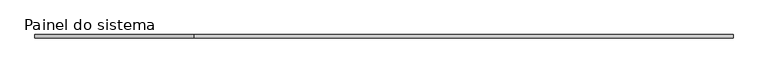
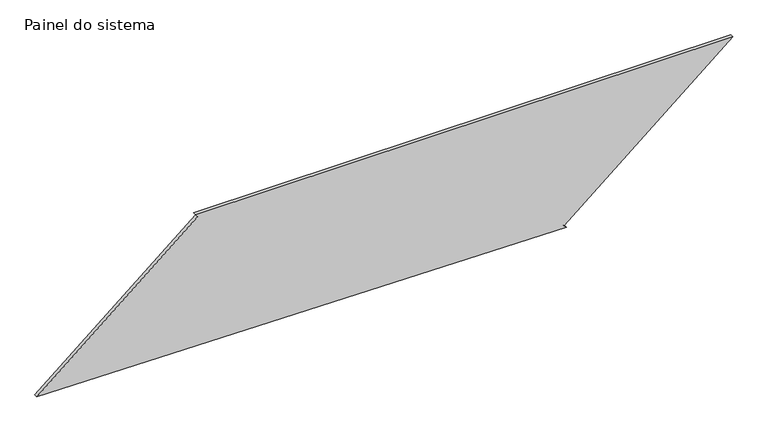
"""IFC4 building model written with IfcOpenShell, lengths in millimetres: plate geometry, Painel do sistema : Envidraçado."""

from ifc_helpers import new_model, si_unit, frame, origin, place, context, project, spatial, polyline, outline, extrude, source, transform, mapped, element, save


def painel_do_sistema_b5e3f343(model_context):
    return source(origin(), model_context, "Body", "SweptSolid", [
        extrude(outline(polyline([(0.0, 1345.1193014), (19.2037959, 1329.1126083), (1059.6226392, 2577.3398982), (1059.6226392, -1401.6658317), (1040.4188433, -1385.6591386), (47.1325024, -2577.3398982), (0.0, 1345.1193014)])), frame((0.0, 24.5, 0.0), z_axis=(0.0, 1.0, 0.0), x_axis=(0.0, 0.0, 1.0)), (0.0, 0.0, 1.0), 25.0),
    ])


if __name__ == "__main__":
    model = new_model("IFC4")
    model_context = context("Model", 3, world=origin())
    ifc_project = project(units=[si_unit("LENGTHUNIT", "METRE", prefix="MILLI")], contexts=[model_context])
    site = spatial("IfcSite", under=ifc_project)
    building = spatial("IfcBuilding", under=site)
    placement = place(None, origin())
    painel_do_sistema_shape = painel_do_sistema_b5e3f343(model_context)
    element("IfcPlate", 1, ObjectType="Painel do sistema : Envidraçado", at=placement, inside=building, context=model_context, shape_type="MappedRepresentation", body=[
        mapped(painel_do_sistema_shape, transform((0.0, 0.0, 0.0), x_axis=(1.0, 0.0, 0.0), y_axis=(0.0, 1.0, 0.0), z_axis=(0.0, 0.0, 1.0))),
    ])
    save(model, "model.ifc")

# Revit data of these elements
# Type "Painel do sistema : Envidraçado"
#   Construction Type Id = "GSP4R"
#   Analytic Construction = "Vidraça única Pilkington 1/8 pol"
#   Visual Light Transmittance = 0.9
#   Solar Heat Gain Coefficient = 0.86
#   Heat Transfer Coefficient (U) = 6.7069 W/(m²·K)
# Element 1 (IfcPlate, "Painel do sistema : Envidraçado")
#   Materials on its faces: "Vidro"
# Materials
#   "Vidro": class "Vidro", colour RGB 0 128 192, transparency 0.9, Description = "Vidro de sílica", Cost = 0
